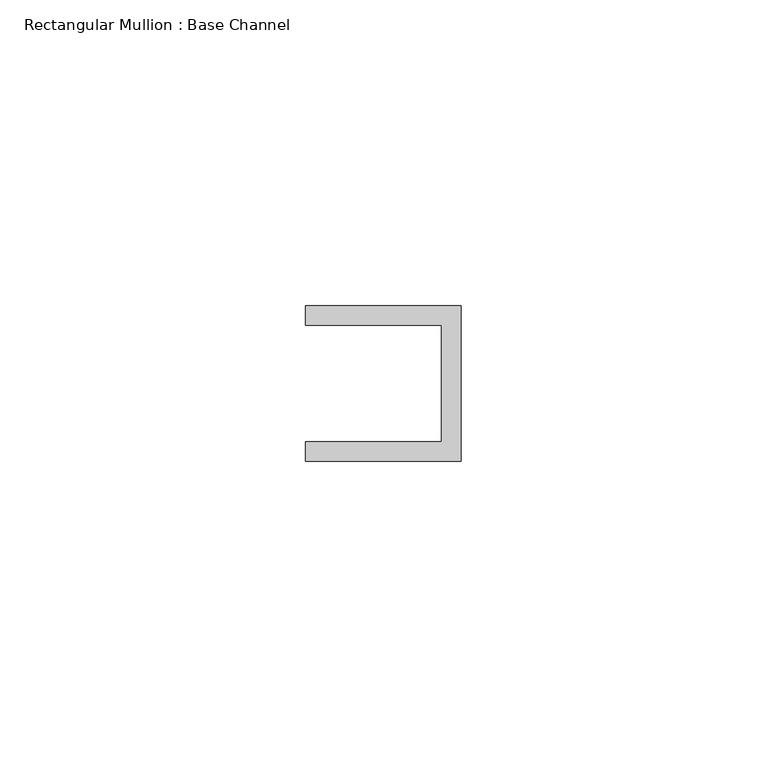
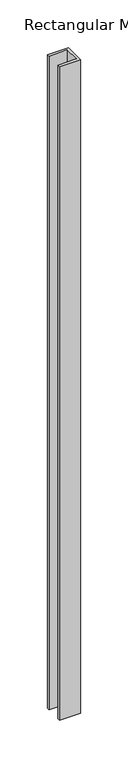
"""IFC4 building model written with IfcOpenShell, lengths in millimetres: member geometry, Rectangular Mullion : Base Channel."""

from ifc_helpers import new_model, si_unit, frame, origin, place, context, project, spatial, polyline, outline, extrude, source, transform, mapped, element, save


def rectangular_mullion_base_channel_0b65783e(model_context):
    return source(origin(), model_context, "Body", "SweptSolid", [
        extrude(outline(polyline([(0.0, -12.7), (-25.4, -12.7), (-25.4, -9.525), (-3.175, -9.525), (-3.175, 9.525), (-25.4, 9.525), (-25.4, 12.7), (0.0, 12.7), (0.0, -12.7)])), frame((0.0, 0.0, -838.2000002), z_axis=(0.0, 0.0, 1.0), x_axis=(1.0, 0.0, 0.0)), (0.0, 0.0, 1.0), 838.2000002),
    ])


if __name__ == "__main__":
    model = new_model("IFC4")
    model_context = context("Model", 3, world=origin())
    ifc_project = project(units=[si_unit("LENGTHUNIT", "METRE", prefix="MILLI")], contexts=[model_context])
    site = spatial("IfcSite", under=ifc_project)
    building = spatial("IfcBuilding", under=site)
    placement = place(None, origin())
    rectangular_mullion_base_channel_shape = rectangular_mullion_base_channel_0b65783e(model_context)
    element("IfcMember", 1, ObjectType="Rectangular Mullion : Base Channel", at=placement, inside=building, context=model_context, shape_type="MappedRepresentation", body=[
        mapped(rectangular_mullion_base_channel_shape, transform((0.0, 0.0, 0.0), x_axis=(1.0, 0.0, 0.0), y_axis=(0.0, 1.0, 0.0), z_axis=(0.0, 0.0, 1.0))),
    ])
    save(model, "model.ifc")

# Revit data of these elements
# Type "Rectangular Mullion : Base Channel"
#   built-in parameter 1007322 = 0.0833333 (stored number, unit not read)
#   built-in parameter 1007321 = 0.0416667 (stored number, unit not read)
#   built-in parameter 1007320 = -0.03125 (stored number, unit not read)
# Element 1 (IfcMember, "Rectangular Mullion : Base Channel")
#   Materials on its faces: "ALUM"
# Materials
#   "ALUM": class "Generic", colour RGB 157 157 157, transparency 0, Cost = 0
